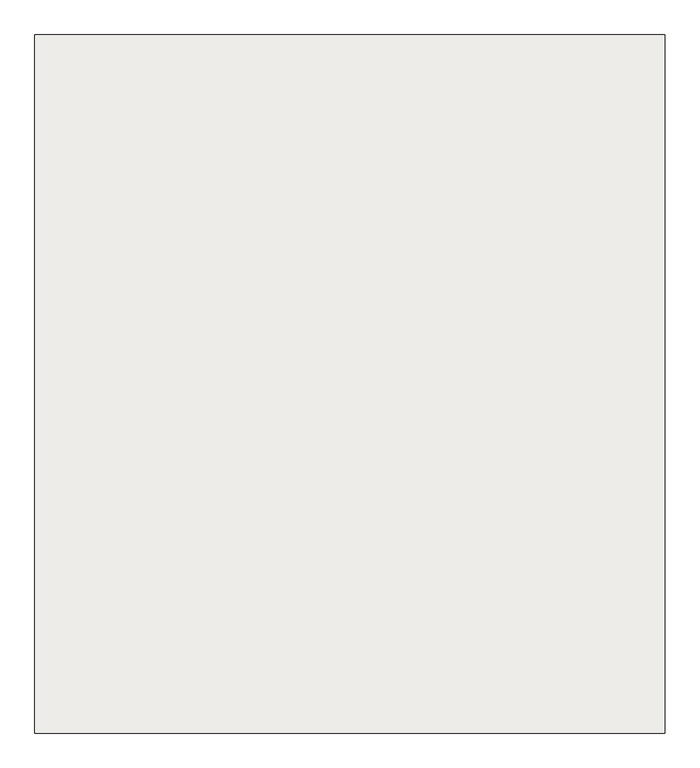
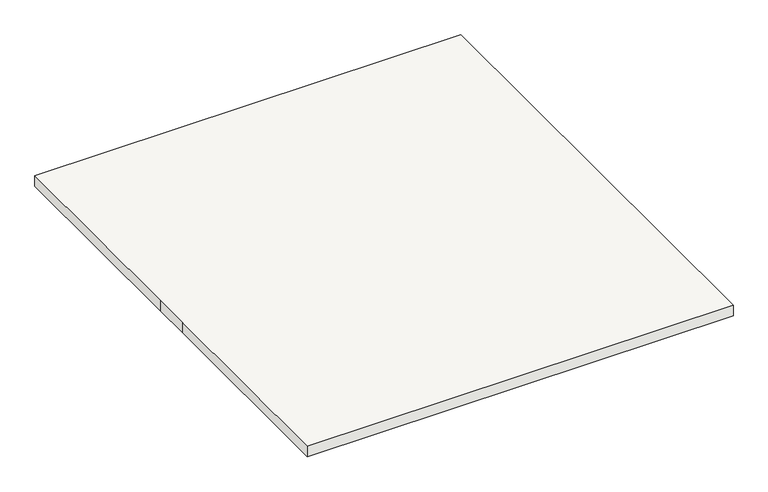
"""IFC4 building model written with IfcOpenShell, lengths in millimetres: slab geometry."""

from ifc_helpers import new_model, si_unit, frame, origin, place, context, project, spatial, polyline, outline, extrude, source, transform, mapped, element, save


def slab_7d48b352(model_context):
    return source(origin(), model_context, "Body", "SweptSolid", [
        extrude(outline(polyline([(5276.5556606, 3685.7983707), (7240.2909543, 3685.7983707), (7240.2909543, 1510.81281), (5276.5556606, 1510.81281), (5276.5556606, 2510.81281), (5276.5556606, 2685.7983707), (5276.5556606, 3685.7983707)])), frame((0.0, 0.0, 1600.0), z_axis=(0.0, 0.0, 1.0), x_axis=(1.0, 0.0, 0.0)), (0.0, 0.0, 1.0), 50.0),
    ])


if __name__ == "__main__":
    model = new_model("IFC4")
    model_context = context("Model", 3, world=origin())
    ifc_project = project(units=[si_unit("LENGTHUNIT", "METRE", prefix="MILLI")], contexts=[model_context])
    site = spatial("IfcSite", under=ifc_project)
    building = spatial("IfcBuilding", under=site)
    placement = place(None, origin())
    slab_shape = slab_7d48b352(model_context)
    element("IfcSlab", 1, at=placement, inside=building, context=model_context, shape_type="MappedRepresentation", body=[
        mapped(slab_shape, transform((0.0, 0.0, 0.0), x_axis=(1.0, 0.0, 0.0), y_axis=(0.0, 1.0, 0.0), z_axis=(0.0, 0.0, 1.0))),
    ])
    save(model, "model.ifc")
